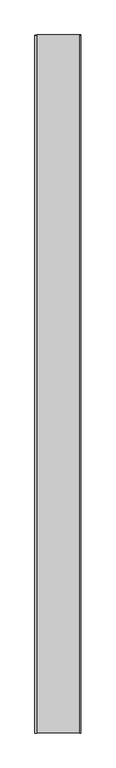
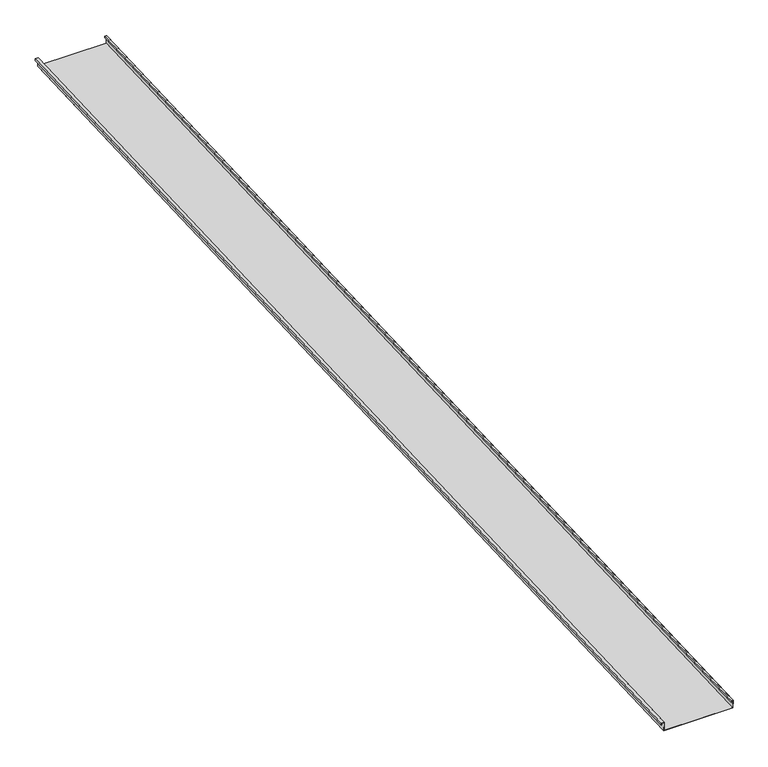
"""IFC4 building model written with IfcOpenShell, lengths in millimetres: proxy geometry, Generic Models 2:Generic Models 2:310765:Generic Models 2:310765 : Generic Models 2:Generic Models 2:310765:105 : Generic Models 2:Generic Models 2:310765:Generic Models 2:310765 : Generic Models 2:Generic Models 2:310765:300385."""

from ifc_helpers import new_model, si_unit, frame, origin, place, context, project, spatial, polyline, outline, extrude, source, transform, mapped, element, save


def generic_models_2d1c399f(model_context):
    return source(origin(), model_context, "Body", "SweptSolid", [
        extrude(outline(polyline([(1.5875, 0.0), (1.5875, 50.8), (407.9875, 50.8), (407.9875, 1.5875), (396.875, 1.5875), (396.875, 11.1125), (398.4625, 11.1125), (398.4625, 3.175), (406.4, 3.175), (406.4, 49.2125), (3.175, 49.2125), (3.175, -1.5874999), (-14.2875, -1.5874999), (-14.2875, 9.525), (-12.7, 9.525), (-12.7, 0.0), (1.5875, 0.0)])), frame((611919.4596406, -581354.4345603, 3902.6697972), z_axis=(0.0, 0.9991330730923568, 0.041630544712067834), x_axis=(1.0, 0.0, 0.0)), (0.0, 0.0, 1.0), 6400.8),
    ])


if __name__ == "__main__":
    model = new_model("IFC4")
    model_context = context("Model", 3, world=origin())
    ifc_project = project(units=[si_unit("LENGTHUNIT", "METRE", prefix="MILLI")], contexts=[model_context])
    site = spatial("IfcSite", under=ifc_project)
    building = spatial("IfcBuilding", under=site)
    placement = place(None, origin())
    generic_models_shape = generic_models_2d1c399f(model_context)
    element("IfcBuildingElementProxy", 1, Name="Generic Models 2:Generic Models 2:310765:Generic Models 2:310765 : Generic Models 2:Generic Models 2:310765:105 : Generic Models 2:Generic Models 2:310765:Generic Models 2:310765 : Generic Models 2:Generic Models 2:310765:300385", ObjectType="Generic Models 2:Generic Models 2:310765:Generic Models 2:310765 : Generic Models 2:Generic Models 2:310765:105 : Generic Models 2:Generic Models 2:310765:Generic Models 2:310765 : Generic Models 2:Generic Models 2:310765:300385", at=placement, inside=building, context=model_context, shape_type="MappedRepresentation", body=[
        mapped(generic_models_shape, transform((0.0, 0.0, 0.0), x_axis=(1.0, 0.0, 0.0), y_axis=(0.0, 1.0, 0.0), z_axis=(0.0, 0.0, 1.0))),
    ])
    save(model, "model.ifc")

# Revit data of these elements
# Type "Generic Models 2:Generic Models 2:310765:Generic Models 2:310765 : Generic Models 2:Generic Models 2:310765:105 : Generic Models 2:Generic Models 2:310765:Generic Models 2:310765 : Generic Models 2:Generic Models 2:310765:300385"
#   NameOverride = "Generic Models 2:Generic Models 2:310765:Generic Models 2:310765 : Generic Models 2:Generic Models 2:310765:300385"
#   ObjectTypeOverride = "Generic Models 2:310765 : Generic Models 2:Generic Models 2:310765"
#   Reference = "Generic Models 2"
#   Tag = "300385"
# Element 1 (IfcBuildingElementProxy, "Generic Models 2:Generic Models 2:310765:Generic Models 2:310765 : Generic Models 2:Generic Models 2:310765:105 : Generic Models 2:Generic Models 2:310765:Generic Models 2:310765 : Generic Models 2:Generic Models 2:310765:300385")
#   Materials on its faces: "THERMAL BROKEN ALUMINUM STOREFRONT FOR POLYCARBONATE"
# Materials
#   "THERMAL BROKEN ALUMINUM STOREFRONT FOR POLYCARBONATE": class "Unassigned", colour RGB 244 244 244, transparency 0, Keynote = "M07611300.01", Cost = 0
